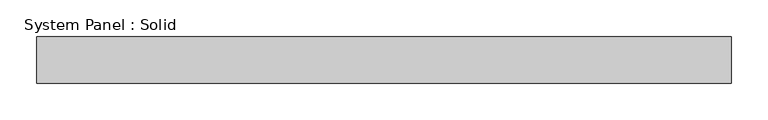
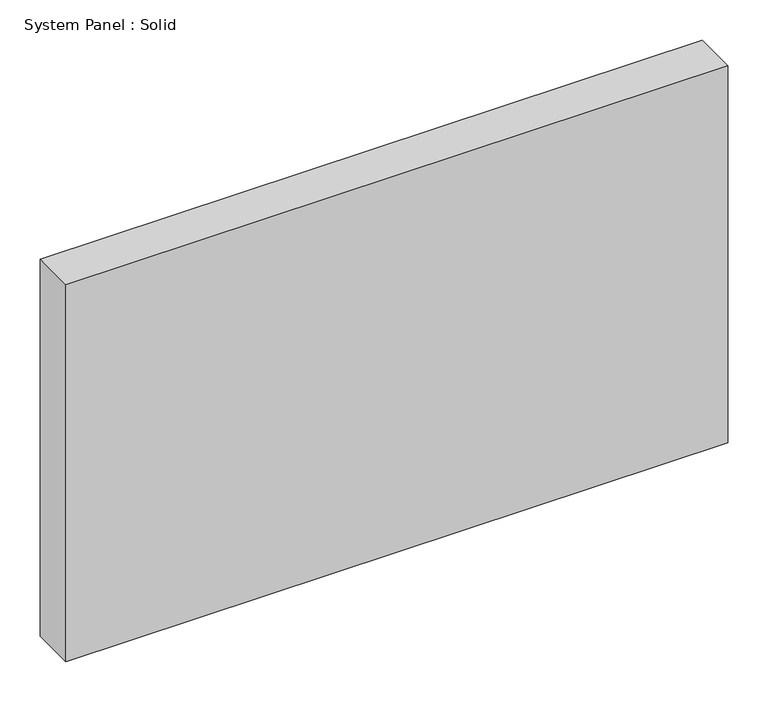
"""IFC4 building model written with IfcOpenShell, lengths in millimetres: plate geometry, System Panel : Solid."""

from ifc_helpers import new_model, si_unit, origin, origin_with_axes, place, context, project, spatial, polyline, outline, extrude, source, transform, mapped, element, save


def system_panel_solid_565455c4(model_context):
    return source(origin(), model_context, "Body", "SweptSolid", [
        extrude(outline(polyline([(474.7095864, -19.05), (-474.7095864, -19.05), (-474.7095864, 44.45), (474.7095864, 44.45), (474.7095864, -19.05)])), origin_with_axes(), (0.0, 0.0, 1.0), 571.5),
    ])


if __name__ == "__main__":
    model = new_model("IFC4")
    model_context = context("Model", 3, world=origin())
    ifc_project = project(units=[si_unit("LENGTHUNIT", "METRE", prefix="MILLI")], contexts=[model_context])
    site = spatial("IfcSite", under=ifc_project)
    building = spatial("IfcBuilding", under=site)
    placement = place(None, origin())
    system_panel_solid_shape = system_panel_solid_565455c4(model_context)
    element("IfcPlate", 1, ObjectType="System Panel : Solid", at=placement, inside=building, context=model_context, shape_type="MappedRepresentation", body=[
        mapped(system_panel_solid_shape, transform((0.0, 0.0, 0.0), x_axis=(1.0, 0.0, 0.0), y_axis=(0.0, 1.0, 0.0), z_axis=(0.0, 0.0, 1.0))),
    ])
    save(model, "model.ifc")

# Revit data of these elements
# Element 1 (IfcPlate, "System Panel : Solid")
#   Materials on its faces: "Default"
# Materials
#   "Default": class "Miscellaneous", colour RGB 127 127 127, transparency 0
